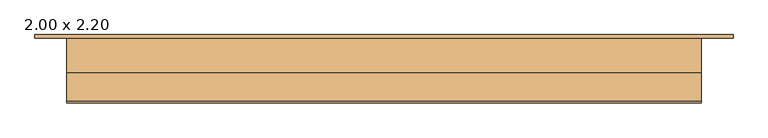
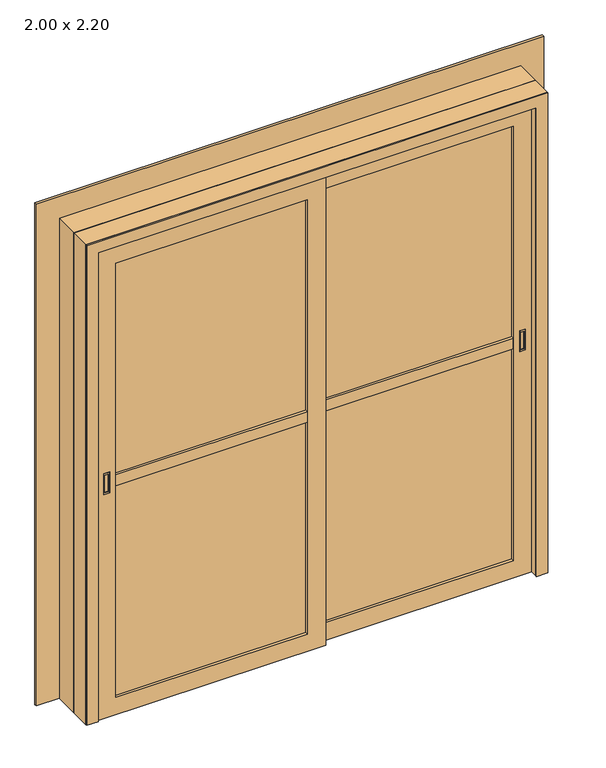
"""IFC4 building model written with IfcOpenShell, lengths in millimetres: door geometry, CC_PORTA CORRER_2 FOLHAS VIDRO : 2.00 x 2.20."""

import ifcopenshell
import ifcopenshell.guid

model = None  # the IFC model being written
_history = None  # IfcOwnerHistory: only IFC2X3 demands one
_inside = {}  # id of a spatial element -> (the spatial element, [elements in it])
_under = {}  # id of a project, library or spatial element -> (it, [spatial elements below it])
_declared = {}  # id of a project -> (the project, [libraries it declares])
_typed = {}  # id of a type object -> (the type object, [elements of that type])
_made_of = {}  # id of a material, layer set ... -> (it, [elements and type objects made of it])


def new_model(schema):
    """Start an empty IFC model of exactly this schema.

    Asked for "IFC4X3", IfcOpenShell would pick the latest addendum, in which some entities
    have other attributes; the version numbers below select the first issue.
    IFC2X3 requires an IfcOwnerHistory on every rooted entity: one is made here for all.
    """
    global model, _history
    if schema == "IFC4X3":
        model = ifcopenshell.file(schema_version=(4, 3, 0, 0))
    else:
        model = ifcopenshell.file(schema=schema)
    _inside.clear()
    _under.clear()
    _declared.clear()
    _typed.clear()
    _made_of.clear()
    _history = None
    if model.schema == "IFC2X3":
        org = make("IfcOrganization", Name="unknown")
        user = make(
            "IfcPersonAndOrganization",
            ThePerson=make("IfcPerson", FamilyName="unknown"),
            TheOrganization=org,
        )
        app = make(
            "IfcApplication",
            ApplicationDeveloper=org,
            Version="unknown",
            ApplicationFullName="unknown",
            ApplicationIdentifier="unknown",
        )
        _history = make(
            "IfcOwnerHistory",
            OwningUser=user,
            OwningApplication=app,
            ChangeAction="ADDED",
            CreationDate=0,
        )
    return model


def make(cls, **values):
    """One entity of the class cls with the attributes given. An attribute that is None is left unset."""
    return model.create_entity(
        cls, **{name: value for name, value in values.items() if value is not None}
    )


def rooted(cls, **values):
    """An entity with a GlobalId (a new one), such as an element, a storey or a relation."""
    return make(cls, GlobalId=ifcopenshell.guid.new(), OwnerHistory=_history, **values)


def si_unit(unit_type, name, prefix=None):
    """IfcSIUnit, for example si_unit("LENGTHUNIT", "METRE", prefix="MILLI")."""
    return make("IfcSIUnit", UnitType=unit_type, Prefix=prefix, Name=name)


def assignment(units):
    """IfcUnitAssignment: the units of a project."""
    return None if units is None else make("IfcUnitAssignment", Units=units)


def point(xyz):
    """IfcCartesianPoint."""
    return None if xyz is None else make("IfcCartesianPoint", Coordinates=xyz)


def direction(xyz):
    """IfcDirection."""
    return None if xyz is None else make("IfcDirection", DirectionRatios=xyz)


def frame(location, z_axis=None, x_axis=None):
    """IfcAxis2Placement3D, a coordinate frame: its origin and axes. An axis left out is left unset."""
    return make(
        "IfcAxis2Placement3D",
        Location=point(location),
        Axis=direction(z_axis),
        RefDirection=direction(x_axis),
    )


def origin():
    """The frame at (0, 0, 0) with its axes left unset."""
    return frame((0.0, 0.0, 0.0))


def place(relative_to, where):
    """IfcLocalPlacement: puts the frame where relative to a parent placement (None: the world)."""
    return make(
        "IfcLocalPlacement", PlacementRelTo=relative_to, RelativePlacement=where
    )


def context(
    kind, dimensions, precision=None, world=None, true_north=None, identifier=None
):
    """IfcGeometricRepresentationContext, for example the 3D "Model" context."""
    return make(
        "IfcGeometricRepresentationContext",
        ContextIdentifier=identifier,
        ContextType=kind,
        CoordinateSpaceDimension=dimensions,
        Precision=precision,
        WorldCoordinateSystem=world,
        TrueNorth=true_north,
    )


def project(units=None, contexts=None):
    """IfcProject with its units and contexts."""
    return rooted(
        "IfcProject",
        Name="project",
        RepresentationContexts=contexts,
        UnitsInContext=assignment(units),
    )


def spatial(cls, under=None, at=None, **own):
    """A site, building, storey or space (cls), placed at a placement, below another one or the project."""
    s = rooted(cls, ObjectPlacement=at, **own)
    if under is not None:
        _under.setdefault(under.id(), (under, []))[1].append(s)
    return s


def polyline(points):
    """IfcPolyline through the points."""
    return make("IfcPolyline", Points=[point(p) for p in points])


def outline(outer, holes=None, kind="AREA"):
    """IfcArbitraryClosedProfileDef: a profile drawn as a closed curve; with holes, ...WithVoids."""
    if holes is None:
        return make("IfcArbitraryClosedProfileDef", ProfileType=kind, OuterCurve=outer)
    return make(
        "IfcArbitraryProfileDefWithVoids",
        ProfileType=kind,
        OuterCurve=outer,
        InnerCurves=holes,
    )


def extrude(swept, where, along, depth):
    """IfcExtrudedAreaSolid: the profile swept, set in the frame where, extruded along a direction by depth."""
    return make(
        "IfcExtrudedAreaSolid",
        SweptArea=swept,
        Position=where,
        ExtrudedDirection=direction(along),
        Depth=depth,
    )


def faces_of(points, faces, orient=None, outer=None):
    """IfcFace entities. A face is a list of loops; a loop is a list of indices into points, from 0.

    orient and outer hold one flag for each loop. By default every Orientation is true, the
    first loop of a face is its IfcFaceOuterBound and the others are IfcFaceBound.
    """
    made = []
    for i, loops in enumerate(faces):
        bounds = []
        for j, loop in enumerate(loops):
            is_outer = j == 0 if outer is None else outer[i][j]
            bounds.append(
                make(
                    "IfcFaceOuterBound" if is_outer else "IfcFaceBound",
                    Bound=make("IfcPolyLoop", Polygon=[points[k] for k in loop]),
                    Orientation=True if orient is None else orient[i][j],
                )
            )
        made.append(make("IfcFace", Bounds=bounds))
    return made


def faceted_brep(points, faces, orient=None, outer=None, voids=None):
    """IfcFacetedBrep: a solid bounded by flat faces; with voids (closed shells), ...WithVoids."""
    shared = [point(p) for p in points]
    hull = make("IfcClosedShell", CfsFaces=faces_of(shared, faces, orient, outer))
    if voids is None:
        return make("IfcFacetedBrep", Outer=hull)
    return make(
        "IfcFacetedBrepWithVoids",
        Outer=hull,
        Voids=[
            make(cls, CfsFaces=faces_of(shared, fs, o, b)) for cls, fs, o, b in voids
        ],
    )


def shape(context_of_items, identifier, shape_type, items):
    """IfcShapeRepresentation: the items that make up one representation, for example the "Body"."""
    return make(
        "IfcShapeRepresentation",
        ContextOfItems=context_of_items,
        RepresentationIdentifier=identifier,
        RepresentationType=shape_type,
        Items=items,
    )


def source(mapping_origin, context_of_items, identifier, shape_type, items):
    """IfcRepresentationMap: a shape defined once, which mapped items show again and again."""
    return make(
        "IfcRepresentationMap",
        MappingOrigin=mapping_origin,
        MappedRepresentation=shape(context_of_items, identifier, shape_type, items),
    )


def transform(
    local_origin,
    x_axis=None,
    y_axis=None,
    z_axis=None,
    scale=None,
    scale2=None,
    scale3=None,
    uniform=True,
):
    """IfcCartesianTransformationOperator3D, or its non-uniform kind. x_axis, y_axis, z_axis: its Axis1, 2, 3."""
    if uniform:
        return make(
            "IfcCartesianTransformationOperator3D",
            Axis1=direction(x_axis),
            Axis2=direction(y_axis),
            LocalOrigin=point(local_origin),
            Scale=scale,
            Axis3=direction(z_axis),
        )
    return make(
        "IfcCartesianTransformationOperator3DnonUniform",
        Axis1=direction(x_axis),
        Axis2=direction(y_axis),
        LocalOrigin=point(local_origin),
        Scale=scale,
        Axis3=direction(z_axis),
        Scale2=scale2,
        Scale3=scale3,
    )


def mapped(mapping_source, mapping_target):
    """IfcMappedItem: shows the shape of a source again, moved by a transform."""
    return make(
        "IfcMappedItem", MappingSource=mapping_source, MappingTarget=mapping_target
    )


def made_of(thing, what):
    """Note that an element or type object is made of a material, layer set ...; save() writes the relation."""
    if what is not None:
        _made_of.setdefault(what.id(), (what, []))[1].append(thing)
    return thing


def element(
    cls,
    number,
    at=None,
    inside=None,
    cuts=None,
    type_object=None,
    material=None,
    context=None,
    identifier="Body",
    shape_type=None,
    held_by="IfcProductDefinitionShape",
    body=None,
    shapes=None,
    **own,
):
    """One element of the class cls, such as IfcWall. Its Tag is "e" and its number.

    at: its placement. inside: the storey or other place that contains it. cuts: it is an
    opening in that element (IfcRelVoidsElement). A single representation is given by context,
    identifier, shape_type and body (its items); several are given by shapes. held_by: the class
    of the entity that holds the representations. save() writes the other relations.
    """
    e = rooted(cls, Tag="e%d" % number, ObjectPlacement=at, **own)
    if body is not None:
        shapes = [shape(context, identifier, shape_type, body)]
    if shapes is not None:
        e.Representation = make(held_by, Representations=shapes)
    if inside is not None:
        _inside.setdefault(inside.id(), (inside, []))[1].append(e)
    if cuts is not None:
        rooted(
            "IfcRelVoidsElement", RelatingBuildingElement=cuts, RelatedOpeningElement=e
        )
    if type_object is not None:
        _typed.setdefault(type_object.id(), (type_object, []))[1].append(e)
    return made_of(e, material)


def aggregate(whole, parts):
    """IfcRelAggregates: a whole, such as a stair, and the parts it consists of."""
    return rooted("IfcRelAggregates", RelatingObject=whole, RelatedObjects=parts)


def save(model, path):
    """Write the relations noted so far, then the file.

    IfcRelAggregates (storeys below a building ...), IfcRelContainedInSpatialStructure (elements
    in a storey), IfcRelDefinesByType, IfcRelAssociatesMaterial and IfcRelDeclares: one each for
    every whole, place, type object, material and project.
    """
    for whole, parts in _under.values():
        aggregate(whole, parts)
    for where, things in _inside.values():
        rooted(
            "IfcRelContainedInSpatialStructure",
            RelatedElements=things,
            RelatingStructure=where,
        )
    for kind, things in _typed.values():
        rooted("IfcRelDefinesByType", RelatedObjects=things, RelatingType=kind)
    for what, things in _made_of.values():
        rooted("IfcRelAssociatesMaterial", RelatedObjects=things, RelatingMaterial=what)
    for by, libraries in _declared.values():
        rooted("IfcRelDeclares", RelatingContext=by, RelatedDefinitions=libraries)
    model.write(path)


def door_2_00_x_2_20_349b5177(model_context):
    return source(origin(), model_context, "Body", "SolidModel", [
        extrude(outline(polyline([(-902.5, -75.0), (-917.5, -75.0), (-917.5, -74.0), (-902.5, -74.0), (-902.5, -75.0)])), frame((0.0, 0.0, 1035.0), z_axis=(0.0, 0.0, 1.0), x_axis=(1.0, 0.0, 0.0)), (0.0, 0.0, 1.0), 80.0),
        extrude(outline(polyline([(1123.0, -897.5), (1123.0, -922.5), (1027.0, -922.5), (1027.0, -897.5), (1123.0, -897.5)]), holes=[polyline([(1115.0, -902.5), (1035.0, -902.5), (1035.0, -917.5), (1115.0, -917.5), (1115.0, -902.5)])]), frame((0.0, -75.0, 0.0), z_axis=(0.0, 1.0, 0.0), x_axis=(0.0, 0.0, 1.0)), (0.0, 0.0, 1.0), 5.1),
        extrude(outline(polyline([(-902.5, -96.0), (-917.5, -96.0), (-917.5, -95.0), (-902.5, -95.0), (-902.5, -96.0)])), frame((0.0, 0.0, 1035.0), z_axis=(0.0, 0.0, 1.0), x_axis=(1.0, 0.0, 0.0)), (0.0, 0.0, 1.0), 80.0),
        extrude(outline(polyline([(1123.0, -897.5), (1123.0, -922.5), (1027.0, -922.5), (1027.0, -897.5), (1123.0, -897.5)]), holes=[polyline([(1115.0, -902.5), (1035.0, -902.5), (1035.0, -917.5), (1115.0, -917.5), (1115.0, -902.5)])]), frame((0.0, -100.1, 0.0), z_axis=(0.0, 1.0, 0.0), x_axis=(0.0, 0.0, 1.0)), (0.0, 0.0, 1.0), 5.1),
        faceted_brep([(-870.0, -70.0, 2070.0), (-870.0, -100.0, 2070.0), (-870.0, -100.0, 80.0), (-870.0, -70.0, 80.0), (-950.0, -100.0, 2150.0), (-950.0, -100.0, 0.0), (40.0, -100.0, 0.0), (40.0, -100.0, 2150.0), (-40.0, -100.0, 2070.0), (-40.0, -100.0, 80.0), (-922.5, -100.0, 1123.0), (-897.5, -100.0, 1123.0), (-897.5, -100.0, 1027.0), (-922.5, -100.0, 1027.0), (-40.0, -70.0, 80.0), (-950.0, -70.0, 0.0), (-950.0, -70.0, 2150.0), (40.0, -70.0, 2150.0), (40.0, -70.0, 0.0), (-40.0, -70.0, 2070.0), (-897.5, -70.0, 1123.0), (-922.5, -70.0, 1123.0), (-922.5, -70.0, 1027.0), (-897.5, -70.0, 1027.0), (-922.5, -95.0, 1123.0), (-897.5, -95.0, 1123.0), (-922.5, -75.0, 1123.0), (-897.5, -75.0, 1123.0), (-897.5, -95.0, 1027.0), (-922.5, -95.0, 1027.0), (-922.5, -75.0, 1027.0), (-897.5, -75.0, 1027.0)], [[[0, 1, 2, 3]], [[4, 5, 6, 7], [2, 1, 8, 9], [10, 11, 12, 13]], [[3, 2, 9, 14]], [[15, 16, 17, 18], [0, 3, 14, 19], [20, 21, 22, 23]], [[4, 16, 15, 5]], [[5, 15, 18, 6]], [[14, 9, 8, 19]], [[6, 18, 17, 7]], [[10, 24, 25, 11]], [[26, 21, 20, 27]], [[11, 25, 28, 12]], [[12, 28, 29, 13]], [[30, 31, 23, 22]], [[24, 10, 13, 29]], [[21, 26, 30, 22]], [[27, 20, 23, 31]], [[25, 24, 29, 28]], [[26, 27, 31, 30]], [[1, 0, 19, 8]], [[16, 4, 7, 17]]]),
        extrude(outline(polyline([(-870.0, -82.0778238), (-40.0, -82.0778238), (-40.0, -87.9221762), (-870.0, -87.9221762), (-870.0, -82.0778238)])), frame((0.0, 0.0, 80.0), z_axis=(0.0, 0.0, 1.0), x_axis=(1.0, 0.0, 0.0)), (0.0, 0.0, 1.0), 1990.0),
        extrude(outline(polyline([(-40.0, -70.0), (-40.0, -100.0), (-870.0, -100.0), (-870.0, -70.0), (-40.0, -70.0)])), frame((0.0, 0.0, 1050.0), z_axis=(0.0, 0.0, 1.0), x_axis=(1.0, 0.0, 0.0)), (0.0, 0.0, 1.0), 50.0),
        extrude(outline(polyline([(902.5, -65.0), (917.5, -65.0), (917.5, -66.0), (902.5, -66.0), (902.5, -65.0)])), frame((0.0, 0.0, 1035.0), z_axis=(0.0, 0.0, 1.0), x_axis=(1.0, 0.0, 0.0)), (0.0, 0.0, 1.0), 80.0),
        extrude(outline(polyline([(1123.0, 897.5), (1027.0, 897.5), (1027.0, 922.5), (1123.0, 922.5), (1123.0, 897.5)]), holes=[polyline([(1115.0, 902.5), (1115.0, 917.5), (1035.0, 917.5), (1035.0, 902.5), (1115.0, 902.5)])]), frame((0.0, -70.1, 0.0), z_axis=(0.0, 1.0, 0.0), x_axis=(0.0, 0.0, 1.0)), (0.0, 0.0, 1.0), 5.1),
        extrude(outline(polyline([(902.5, -44.0), (917.5, -44.0), (917.5, -45.0), (902.5, -45.0), (902.5, -44.0)])), frame((0.0, 0.0, 1035.0), z_axis=(0.0, 0.0, 1.0), x_axis=(1.0, 0.0, 0.0)), (0.0, 0.0, 1.0), 80.0),
        extrude(outline(polyline([(1123.0, 897.5), (1027.0, 897.5), (1027.0, 922.5), (1123.0, 922.5), (1123.0, 897.5)]), holes=[polyline([(1115.0, 902.5), (1115.0, 917.5), (1035.0, 917.5), (1035.0, 902.5), (1115.0, 902.5)])]), frame((0.0, -45.0, 0.0), z_axis=(0.0, 1.0, 0.0), x_axis=(0.0, 0.0, 1.0)), (0.0, 0.0, 1.0), 5.1),
        faceted_brep([(870.0, -70.0, 2070.0), (870.0, -40.0, 2070.0), (870.0, -40.0, 80.0), (870.0, -70.0, 80.0), (950.0, -40.0, 2150.0), (950.0, -40.0, 0.0), (-40.0, -40.0, 0.0), (-40.0, -40.0, 2150.0), (40.0, -40.0, 2070.0), (40.0, -40.0, 80.0), (922.5, -40.0, 1123.0), (897.5, -40.0, 1123.0), (897.5, -40.0, 1027.0), (922.5, -40.0, 1027.0), (40.0, -70.0, 80.0), (950.0, -70.0, 0.0), (950.0, -70.0, 2150.0), (-40.0, -70.0, 2150.0), (-40.0, -70.0, 0.0), (40.0, -70.0, 2070.0), (897.5, -70.0, 1123.0), (922.5, -70.0, 1123.0), (922.5, -70.0, 1027.0), (897.5, -70.0, 1027.0), (922.5, -45.0, 1123.0), (897.5, -45.0, 1123.0), (922.5, -65.0, 1123.0), (897.5, -65.0, 1123.0), (897.5, -45.0, 1027.0), (922.5, -45.0, 1027.0), (922.5, -65.0, 1027.0), (897.5, -65.0, 1027.0)], [[[0, 1, 2, 3]], [[4, 5, 6, 7], [2, 1, 8, 9], [10, 11, 12, 13]], [[3, 2, 9, 14]], [[15, 16, 17, 18], [0, 3, 14, 19], [20, 21, 22, 23]], [[4, 16, 15, 5]], [[5, 15, 18, 6]], [[14, 9, 8, 19]], [[6, 18, 17, 7]], [[10, 24, 25, 11]], [[26, 21, 20, 27]], [[11, 25, 28, 12]], [[12, 28, 29, 13]], [[30, 31, 23, 22]], [[24, 10, 13, 29]], [[21, 26, 30, 22]], [[27, 20, 23, 31]], [[25, 24, 29, 28]], [[26, 27, 31, 30]], [[1, 0, 19, 8]], [[16, 4, 7, 17]]]),
        extrude(outline(polyline([(870.0, -57.9221762), (40.0, -57.9221762), (40.0, -52.0778238), (870.0, -52.0778238), (870.0, -57.9221762)])), frame((0.0, 0.0, 80.0), z_axis=(0.0, 0.0, 1.0), x_axis=(1.0, 0.0, 0.0)), (0.0, 0.0, 1.0), 1990.0),
        extrude(outline(polyline([(40.0, -70.0), (40.0, -40.0), (870.0, -40.0), (870.0, -70.0), (40.0, -70.0)])), frame((0.0, 0.0, 1050.0), z_axis=(0.0, 0.0, 1.0), x_axis=(1.0, 0.0, 0.0)), (0.0, 0.0, 1.0), 50.0),
        extrude(outline(polyline([(0.0, -1000.0), (0.0, -950.0), (2150.0, -950.0), (2150.0, 950.0), (0.0, 950.0), (0.0, 1000.0), (2200.0, 1000.0), (2200.0, -1000.0), (0.0, -1000.0)])), frame((0.0, -105.0, 0.0), z_axis=(0.0, 1.0, 0.0), x_axis=(0.0, 0.0, 1.0)), (0.0, 0.0, 1.0), 5.0),
        faceted_brep([(999.0, 110.0, 0.0), (1100.0, 110.0, 0.0), (1100.0, 100.0, 0.0), (1000.0, 100.0, 0.0), (1000.0, -10.0, 0.0), (999.0, -10.0, 0.0), (999.0, 110.0, 2199.0), (-999.0, 110.0, 2199.0), (-999.0, 110.0, 0.0), (-1100.0, 110.0, 0.0), (-1100.0, 110.0, 2300.0), (1100.0, 110.0, 2300.0), (1100.0, 100.0, 2300.0), (-1100.0, 100.0, 2300.0), (-1100.0, 100.0, 0.0), (-1000.0, 100.0, 0.0), (-1000.0, 100.0, 2200.0), (1000.0, 100.0, 2200.0), (1000.0, -10.0, 2200.0), (-1000.0, -10.0, 2200.0), (-1000.0, -10.0, 0.0), (-999.0, -10.0, 0.0), (-999.0, -10.0, 2199.0), (999.0, -10.0, 2199.0)], [[[0, 1, 2, 3, 4, 5]], [[1, 0, 6, 7, 8, 9, 10, 11]], [[2, 1, 11, 12]], [[3, 2, 12, 13, 14, 15, 16, 17]], [[4, 3, 17, 18]], [[5, 4, 18, 19, 20, 21, 22, 23]], [[0, 5, 23, 6]], [[8, 21, 20, 15, 14, 9]], [[7, 22, 21, 8]], [[19, 16, 15, 20]], [[13, 10, 9, 14]], [[12, 11, 10, 13]], [[18, 17, 16, 19]], [[6, 23, 22, 7]]]),
        extrude(outline(polyline([(0.0, -1000.0), (0.0, -950.0), (2150.0, -950.0), (2150.0, 950.0), (0.0, 950.0), (0.0, 1000.0), (2200.0, 1000.0), (2200.0, -1000.0), (0.0, -1000.0)])), frame((0.0, -100.0, 0.0), z_axis=(0.0, 1.0, 0.0), x_axis=(0.0, 0.0, 1.0)), (0.0, 0.0, 1.0), 90.0),
    ])


if __name__ == "__main__":
    model = new_model("IFC4")
    model_context = context("Model", 3, world=origin())
    ifc_project = project(units=[si_unit("LENGTHUNIT", "METRE", prefix="MILLI")], contexts=[model_context])
    site = spatial("IfcSite", under=ifc_project)
    building = spatial("IfcBuilding", under=site)
    placement = place(None, origin())
    door_2_00_x_2_20_shape = door_2_00_x_2_20_349b5177(model_context)
    element("IfcDoor", 1, ObjectType="CC_PORTA CORRER_2 FOLHAS VIDRO : 2.00 x 2.20", at=placement, inside=building, context=model_context, shape_type="MappedRepresentation", body=[
        mapped(door_2_00_x_2_20_shape, transform((0.0, 0.0, 0.0), x_axis=(1.0, 0.0, 0.0), y_axis=(0.0, 1.0, 0.0), z_axis=(0.0, 0.0, 1.0))),
    ])
    save(model, "model.ifc")

# Revit data of these elements
# Type "CC_PORTA CORRER_2 FOLHAS VIDRO : 2.00 x 2.20"
#   Type Mark = "PV2"
#   Site = "www.construir.arq.br"
#   Empresa = "Cursos Construir"
#   Criado Por = "Roberto Netto"
#   Analytic Construction = "<Nenhum>"
#   Rough Width = 2.00 m
#   Largura Moldura Folha [instance default] = 0.08 m
#   Largura Barra Central Folha [instance default] = 0.05 m
#   Largura Guarnição Interna [instance default] = 0.05 m
#   Largura Moldura Externa [instance default] = 0.10 m
#   Largura Folha [instance default] = 0.99 m
#   Interna [instance default] = 0.00 m
#   Externa [instance default] = 0.00 m
#   Extensão Lateral Esquerda [instance default] = 0.03 m
#   Extensão Frontal [instance default] = 0.03 m
#   Extensão Batente [instance default] = 0.03 m
#   Extensão Lateral Direita [instance default] = 0.03 m
#   Espessura Soleira [instance default] = 0.02 m
#   Espessura Guarnição Interna [instance default] = 0.005 m
#   Espessura Moldura Externa [instance default] = 0.01 m
#   Espessura Folha [instance default] = 0.03 m
#   Espessura Batente [instance default] = 0.05 m
#   Desloc Interno [instance default] = 0.00 m
#   Rough Height = 2.20 m
#   Altura Folha [instance default] = 2.15 m
#   Height = 2.20 m
#   Width = 2.00 m
#   ----SOLEIRA---- [instance default] = 0.00 m
#   ----MOLDURA---- [instance default] = 0.00 m
#   ----GUARNIÇÃO---- [instance default] = 0.00 m
#   ----FOLHA---- [instance default] = 0.00 m
#   ----EXTENSÃO---- [instance default] = 0.00 m
#   ----BATENTE---- [instance default] = 0.00 m
#   Soleira Sem Extensão [instance default] = yes
#   Soleira Com Extensão [instance default] = no
#   Soleira [instance default] = yes
#   Puxador [instance default] = yes
#   Porcent. Exibição Batente Interno [instance default] = 0
#   Moldura Externa [instance default] = yes
#   Guarnição Interna [instance default] = yes
#   Function = 1
#   Barra Central [instance default] = yes
#   Material Vidro Folha = .VIDRO
#   Material Soleira = .GRANITO BRANCO ITAÚNAS
#   Material Puxador = .ALUMÍNIO COM PINTURA ELETROSTÁTICA BRANCA
#   Material Moldura Externa = .PINTURA ACRÍLICA BRANCA
#   Material Moldura Folha = .ALUMÍNIO COM PINTURA ELETROSTÁTICA BRANCA
#   Material Guarnição Interna = .ALUMÍNIO COM PINTURA ELETROSTÁTICA BRANCA
#   Material Batente = .ALUMÍNIO COM PINTURA ELETROSTÁTICA BRANCA
#   Wall Closure = (empty or 0)
# Element 1 (IfcDoor, "CC_PORTA CORRER_2 FOLHAS VIDRO : 2.00 x 2.20")
#   Materials on its faces: ".ALUMÍNIO COM PINTURA ELETROSTÁTICA BRANCA", ".PINTURA ACRÍLICA BRANCA", ".VIDRO"
# Materials
#   ".VIDRO": class "Genérico", colour RGB 198 236 255, transparency 0.95, Cost = 0
#   ".GRANITO BRANCO ITAÚNAS": class ".CC_PEDRA REVEST.", colour RGB 202 195 174, transparency 0, Description = "Granito branco Itaúnas", Uso = "Pedra", Cost = 0
#   ".ALUMÍNIO COM PINTURA ELETROSTÁTICA BRANCA": class "CC_METAIS", colour RGB 241 241 241, transparency 0, Cost = 0
#   ".PINTURA ACRÍLICA BRANCA": class ".CC_PINTURA", colour RGB 250 250 250, transparency 0, Keynote = "09910.A1", Description = "Tinta acrílica na cor branca", Cost = 0
